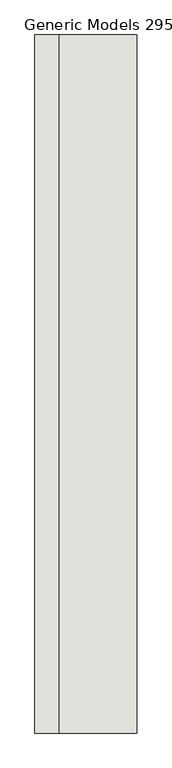
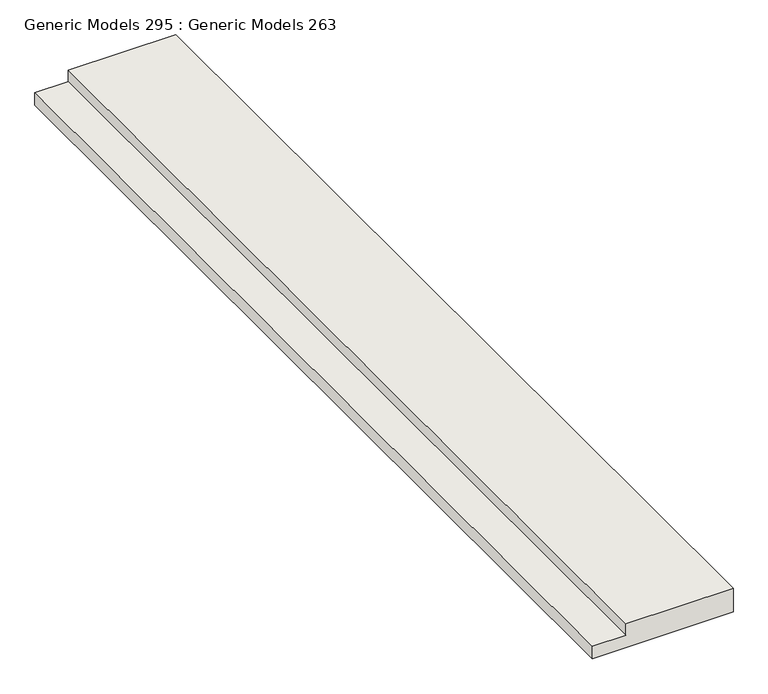
"""IFC4 building model written with IfcOpenShell, lengths in millimetres: wall geometry, Generic Models 295 : Generic Models 263."""

from ifc_helpers import new_model, si_unit, frame, origin, place, context, project, spatial, polyline, outline, extrude, source, transform, mapped, element, save


def generic_models_295_generic_models_263_c61a579b(model_context):
    return source(origin(), model_context, "Body", "SweptSolid", [
        extrude(outline(polyline([(-381.0, 92037.1797726), (-381.0, 91579.9797726), (-558.8, 91579.9797726), (-558.8, 93498.3966125), (-215.9, 93498.3966125), (-215.9, 92037.1797726), (-381.0, 92037.1797726)])), frame((0.0, -9654.0595125, 0.0), z_axis=(0.0, 1.0, 0.0), x_axis=(0.0, 0.0, 1.0)), (0.0, 0.0, 1.0), 13158.0645094),
    ])


if __name__ == "__main__":
    model = new_model("IFC4")
    model_context = context("Model", 3, world=origin())
    ifc_project = project(units=[si_unit("LENGTHUNIT", "METRE", prefix="MILLI")], contexts=[model_context])
    site = spatial("IfcSite", under=ifc_project)
    building = spatial("IfcBuilding", under=site)
    placement = place(None, origin())
    generic_models_295_generic_models_263_shape = generic_models_295_generic_models_263_c61a579b(model_context)
    element("IfcWall", 1, ObjectType="Generic Models 295 : Generic Models 263", at=placement, inside=building, context=model_context, shape_type="MappedRepresentation", body=[
        mapped(generic_models_295_generic_models_263_shape, transform((0.0, 0.0, 0.0), x_axis=(1.0, 0.0, 0.0), y_axis=(0.0, 1.0, 0.0), z_axis=(0.0, 0.0, 1.0))),
    ])
    save(model, "model.ifc")

# Revit data of these elements
# Element 1 (IfcWall, "Generic Models 295 : Generic Models 263")
#   Materials on its faces: "CRUSHED AGGREGATE BASE COURSE"
# Materials
#   "CRUSHED AGGREGATE BASE COURSE": class "Miscellaneous", colour RGB 183 184 198, transparency 0, Cost = 0
